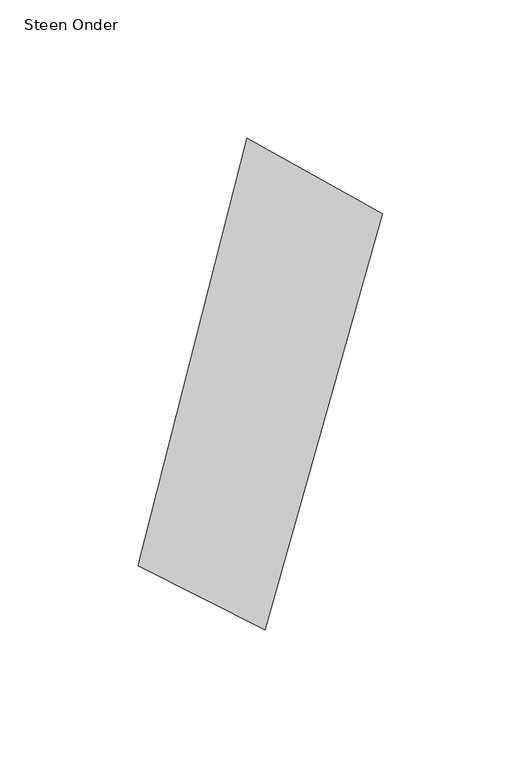
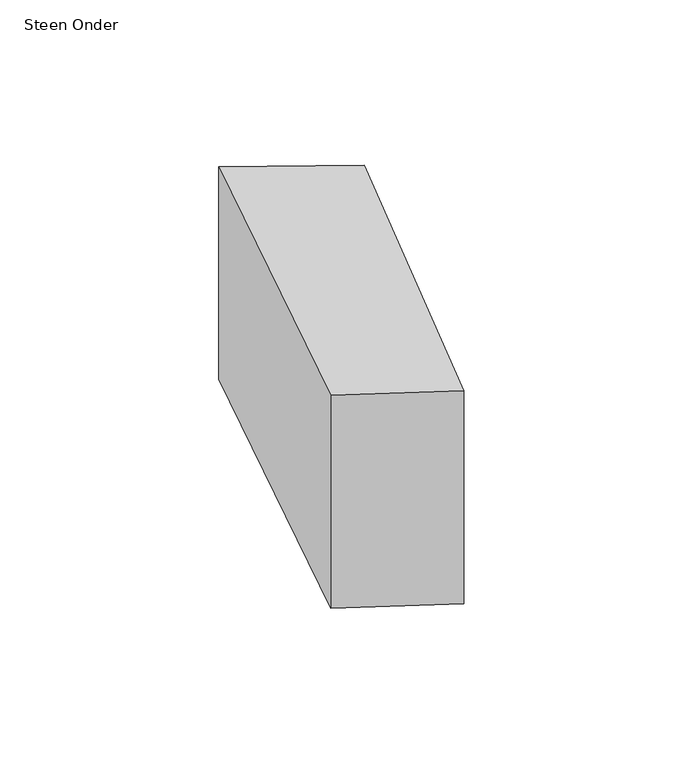
"""IFC4 building model written with IfcOpenShell, lengths in millimetres: proxy geometry, 00_GMA_steen_versie_4 : Steen Onder."""

from ifc_helpers import new_model, si_unit, origin, origin_with_axes, place, context, project, spatial, polyline, outline, extrude, source, transform, mapped, element, save


def steen_onder_19602b1c(model_context):
    return source(origin(), model_context, "Body", "SweptSolid", [
        extrude(outline(polyline([(121.7635088, 143.7279899), (79.1952797, -6.5708087), (33.4127485, 16.5591785), (72.7583362, 170.9963354), (121.7635088, 143.7279899)])), origin_with_axes(), (0.0, 0.0, 1.0), 100.0),
    ])


if __name__ == "__main__":
    model = new_model("IFC4")
    model_context = context("Model", 3, world=origin())
    ifc_project = project(units=[si_unit("LENGTHUNIT", "METRE", prefix="MILLI")], contexts=[model_context])
    site = spatial("IfcSite", under=ifc_project)
    building = spatial("IfcBuilding", under=site)
    placement = place(None, origin())
    steen_onder_shape = steen_onder_19602b1c(model_context)
    element("IfcBuildingElementProxy", 1, Name="00_GMA_steen_versie_4 : Steen Onder", ObjectType="00_GMA_steen_versie_4 : Steen Onder", at=placement, inside=building, context=model_context, shape_type="MappedRepresentation", body=[
        mapped(steen_onder_shape, transform((0.0, 0.0, 0.0), x_axis=(1.0, 0.0, 0.0), y_axis=(0.0, 1.0, 0.0), z_axis=(0.0, 0.0, 1.0))),
    ])
    save(model, "model.ifc")

# Revit data of these elements
# Type "00_GMA_steen_versie_4 : Steen Onder"
#   StootVoegHalfBoven [instance default] = 5 mm
#   StootVoegHalf [instance default] = 5 mm
#   StootVoegBreedteOnder = 10 mm
#   StootVoegBreedteBoven = 10 mm
#   Steendikte = 100 mm
#   LintVoegOnderHalf = 0 mm
#   LintVoegOnder = 0 mm
#   LintVoegBovenHalf = 5 mm
#   LintVoegBoven = 10 mm
#   materiaal = none
#   MateriaalVoeg = none
#   Default Elevation = 0
